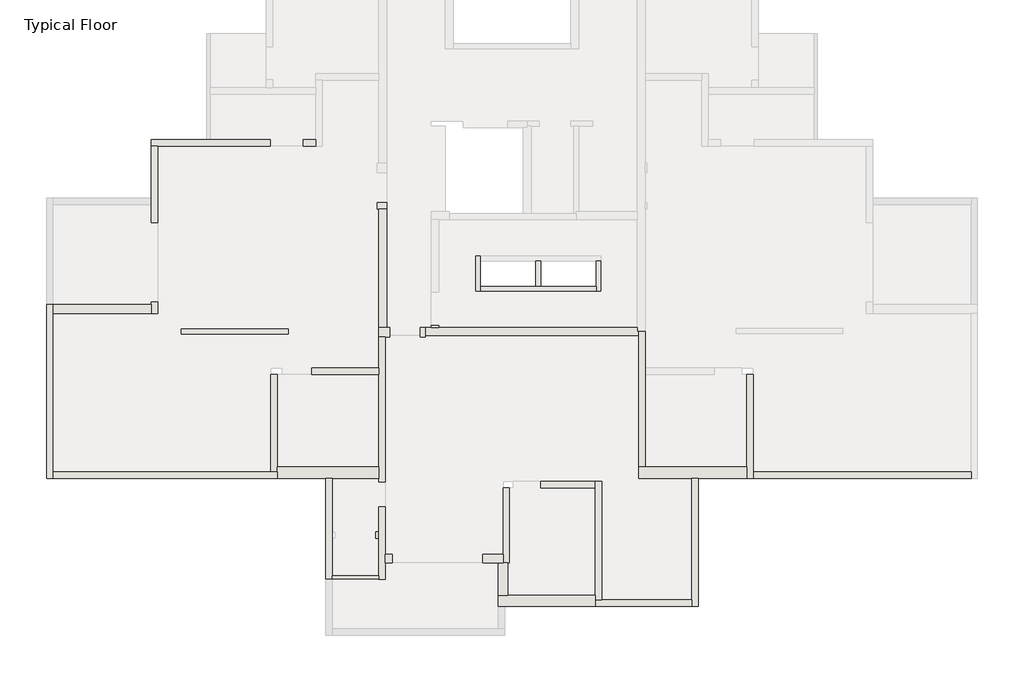
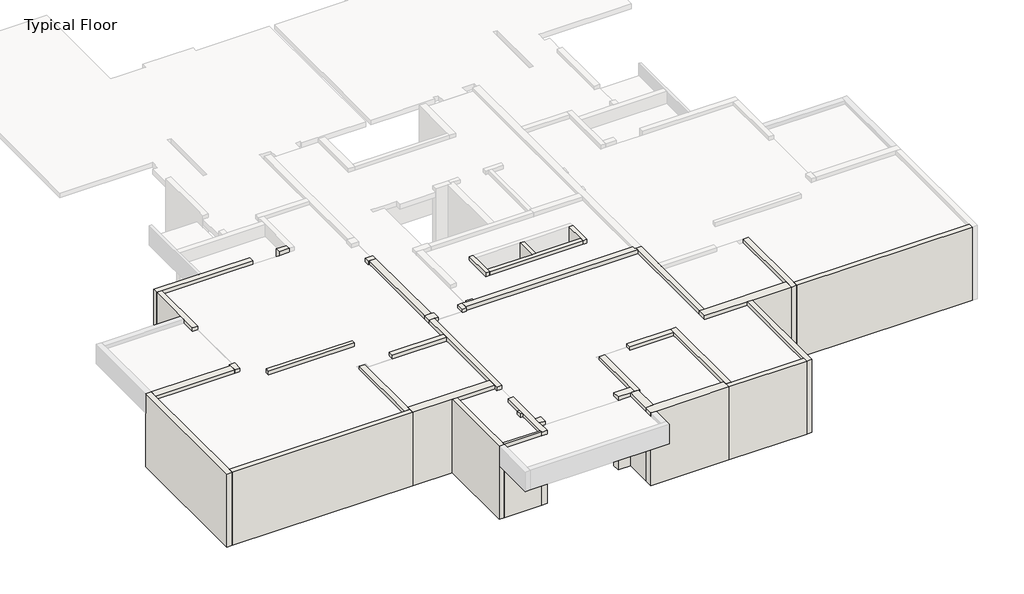
# One storey, part 1 of 4: 39 walls.
"""IFC4 building model written with IfcOpenShell, lengths in millimetres."""

from ifc_helpers import new_model, si_unit, frame, origin, place, context, project, spatial, polyline, outline, extrude, faceted_brep, element, save

model = new_model("IFC4")

# Units and contexts
model_context = context("Model", 3, world=origin())
ifc_project = project(units=[si_unit("LENGTHUNIT", "METRE", prefix="MILLI")], contexts=[model_context])

# Site, building, storey
site = spatial("IfcSite", under=ifc_project)
building = spatial("IfcBuilding", under=site)
storey = spatial("IfcBuildingStorey", under=building, Name="Typical Floor", Elevation=3160.0)

# Walls
placement = place(None, origin())
element("IfcWall", 1, ObjectType="10", at=placement, inside=storey, context=model_context, shape_type="Brep", body=[
    faceted_brep([(-1104.0660316, -14027.6329213, 160.0), (353.6524939, -14027.6329213, 160.0), (353.6524939, -14027.6329213, 2810.0), (353.6524939, -14027.6329213, 3010.0), (353.6524939, -14027.6329213, 3160.0), (-1104.0660316, -14027.6329213, 3160.0), (-1104.0660316, -14027.6329213, 3010.0), (-1104.0660316, -14027.6329213, 2810.0), (-1104.0660316, -13927.6329213, 160.0), (-1104.0660316, -13927.6329213, 3160.0), (353.6524939, -13927.6329213, 3160.0), (353.6524939, -13927.6329213, 3010.0), (353.6524939, -13927.6329213, 2810.0), (353.6524939, -13927.6329213, 160.0)], [[[0, 1, 2, 3, 4, 5, 6, 7]], [[8, 9, 10, 11, 12, 13]], [[1, 0, 8, 13]], [[5, 4, 10, 9]], [[4, 3, 2, 1, 13, 12, 11, 10]], [[0, 7, 6, 5, 9, 8]]]),
])
element("IfcWall", 2, ObjectType="15", at=placement, inside=storey, context=model_context, shape_type="Brep", body=[
    faceted_brep([(-5822.171691, -6349.5529829, 160.0), (-2483.2956212, -6349.5529829, 160.0), (-2483.2956212, -6349.5529829, 2810.0), (-2483.2956212, -6349.5529829, 3010.0), (-2483.2956212, -6349.5529829, 3160.0), (-5822.171691, -6349.5529829, 3160.0), (-5822.171691, -6349.5529829, 3010.0), (-5822.171691, -6349.5529829, 2810.0), (-5822.171691, -6199.5529829, 160.0), (-5822.171691, -6199.5529829, 2810.0), (-5822.171691, -6199.5529829, 3010.0), (-5822.171691, -6199.5529829, 3160.0), (-2483.2956212, -6199.5529829, 3160.0), (-2483.2956212, -6199.5529829, 3010.0), (-2483.2956212, -6199.5529829, 2810.0), (-2483.2956212, -6199.5529829, 160.0)], [[[0, 1, 2, 3, 4, 5, 6, 7]], [[8, 9, 10, 11, 12, 13, 14, 15]], [[1, 0, 8, 15]], [[4, 3, 2, 1, 15, 14, 13, 12]], [[5, 4, 12, 11]], [[0, 7, 6, 5, 11, 10, 9, 8]]]),
])
element("IfcWall", 3, ObjectType="15", at=placement, inside=storey, context=model_context, shape_type="Brep", body=[
    faceted_brep([(3535.5549057, -5009.2269053, 160.0), (3535.5549057, -4859.2269053, 160.0), (3535.5549057, -4065.4538564, 160.0), (3535.5549057, -3915.4538564, 160.0), (3535.5549057, -3915.4538564, 3160.0), (3535.5549057, -4065.4538564, 3160.0), (3535.5549057, -4859.2269053, 3160.0), (3535.5549057, -5009.2269053, 3160.0), (3385.5549057, -5009.2269053, 160.0), (3385.5549057, -5009.2269053, 2810.0), (3385.5549057, -5009.2269053, 3010.0), (3385.5549057, -5009.2269053, 3160.0), (3385.5549057, -3915.4538564, 3160.0), (3385.5549057, -3915.4538564, 3010.0), (3385.5549057, -3915.4538564, 2810.0), (3385.5549057, -3915.4538564, 160.0)], [[[0, 1, 2, 3, 4, 5, 6, 7]], [[8, 9, 10, 11, 12, 13, 14, 15]], [[3, 2, 1, 0, 8, 15]], [[7, 6, 5, 4, 12, 11]], [[4, 3, 15, 14, 13, 12]], [[0, 7, 11, 10, 9, 8]]]),
])
element("IfcWall", 4, ObjectType="15", at=placement, inside=storey, context=model_context, shape_type="Brep", body=[
    faceted_brep([(7154.2538596, -4065.4538564, 160.0), (7154.2538596, -4859.2269053, 160.0), (7154.2538596, -5009.2269053, 160.0), (7154.2538596, -5009.2269053, 3160.0), (7154.2538596, -4859.2269053, 3160.0), (7154.2538596, -4065.4538564, 3160.0), (7304.2538596, -4065.4538564, 160.0), (7304.2538596, -4065.4538564, 3160.0), (7304.2538596, -5009.2269053, 3160.0), (7304.2538596, -5009.2269053, 3010.0), (7304.2538596, -5009.2269053, 2810.0), (7304.2538596, -5009.2269053, 160.0)], [[[0, 1, 2, 3, 4, 5]], [[6, 7, 8, 9, 10, 11]], [[2, 1, 0, 6, 11]], [[5, 4, 3, 8, 7]], [[0, 5, 7, 6]], [[3, 2, 11, 10, 9, 8]]]),
])
element("IfcWall", 5, ObjectType="15", at=placement, inside=storey, context=model_context, shape_type="Brep", body=[
    faceted_brep([(7154.2538596, -4859.2269053, 160.0), (5418.6420666, -4859.2269053, 160.0), (5268.6420666, -4859.2269053, 160.0), (3535.5549057, -4859.2269053, 160.0), (3535.5549057, -4859.2269053, 3160.0), (5268.6420666, -4859.2269053, 3160.0), (5418.6420666, -4859.2269053, 3160.0), (7154.2538596, -4859.2269053, 3160.0), (7154.2538596, -5009.2269053, 160.0), (7154.2538596, -5009.2269053, 3160.0), (3535.5549057, -5009.2269053, 3160.0), (3535.5549057, -5009.2269053, 160.0)], [[[0, 1, 2, 3, 4, 5, 6, 7]], [[8, 9, 10, 11]], [[3, 2, 1, 0, 8, 11]], [[7, 6, 5, 4, 10, 9]], [[0, 7, 9, 8]], [[4, 3, 11, 10]]]),
])
element("IfcWall", 6, ObjectType="15", at=placement, inside=storey, context=model_context, shape_type="SweptSolid", body=[
    extrude(outline(polyline([(5418.6420666, -4065.4538564), (5418.6420666, -4859.2269053), (5268.6420666, -4859.2269053), (5268.6420666, -4065.4538564), (5418.6420666, -4065.4538564)])), frame((0.0, 0.0, 160.0), z_axis=(0.0, 0.0, 1.0), x_axis=(1.0, 0.0, 0.0)), (0.0, 0.0, 1.0), 3000.0),
])
element("IfcWall", 7, ObjectType="20", at=placement, inside=storey, context=model_context, shape_type="Brep", body=[
    faceted_brep([(10348.1730809, -14884.0133443, 160.0), (10348.1730809, -10869.1739201, 160.0), (10348.1730809, -10869.1739201, 3160.0), (10348.1730809, -14884.0133443, 3160.0), (10148.1730809, -14884.0133443, 160.0), (10148.1730809, -14884.0133443, 3160.0), (10148.1730809, -14684.0133443, 3160.0), (10148.1730809, -10869.1739201, 3160.0), (10148.1730809, -10869.1739201, 3010.0), (10148.1730809, -10869.1739201, 2810.0), (10148.1730809, -10869.1739201, 160.0), (10148.1730809, -14684.0133443, 160.0)], [[[0, 1, 2, 3]], [[4, 5, 6, 7, 8, 9, 10, 11]], [[1, 0, 4, 11, 10]], [[3, 2, 7, 6, 5]], [[2, 1, 10, 9, 8, 7]], [[0, 3, 5, 4]]]),
])
element("IfcWall", 8, ObjectType="20", at=placement, inside=storey, context=model_context, shape_type="Brep", body=[
    faceted_brep([(10148.1730809, -14684.0133443, 160.0), (7323.2436151, -14684.0133443, 160.0), (7123.2436151, -14684.0133443, 160.0), (7123.2436151, -14684.0133443, 3160.0), (7323.2436151, -14684.0133443, 3160.0), (10148.1730809, -14684.0133443, 3160.0), (10148.1730809, -14684.0133443, 3010.0), (10148.1730809, -14684.0133443, 2810.0), (10148.1730809, -14884.0133443, 160.0), (10148.1730809, -14884.0133443, 3160.0), (7123.2436151, -14884.0133443, 3160.0), (7123.2436151, -14884.0133443, 160.0)], [[[0, 1, 2, 3, 4, 5, 6, 7]], [[8, 9, 10, 11]], [[2, 1, 0, 8, 11]], [[5, 4, 3, 10, 9]], [[3, 2, 11, 10]], [[0, 7, 6, 5, 9, 8]]]),
])
element("IfcWall", 9, ObjectType="20", at=placement, inside=storey, context=model_context, shape_type="Brep", body=[
    faceted_brep([(7323.2436151, -14684.0133443, 160.0), (7323.2436151, -10973.6256761, 160.0), (7323.2436151, -10973.6256761, 2810.0), (7323.2436151, -10973.6256761, 3010.0), (7323.2436151, -10973.6256761, 3160.0), (7323.2436151, -14684.0133443, 3160.0), (7323.2436151, -14684.0133443, 3010.0), (7323.2436151, -14684.0133443, 2810.0), (7123.2436151, -14684.0133443, 160.0), (7123.2436151, -14684.0133443, 3160.0), (7123.2436151, -14534.0137597, 3160.0), (7123.2436151, -11173.6256761, 3160.0), (7123.2436151, -10973.6256761, 3160.0), (7123.2436151, -10973.6256761, 160.0), (7123.2436151, -11173.6256761, 160.0), (7123.2436151, -14534.0137597, 160.0)], [[[0, 1, 2, 3, 4, 5, 6, 7]], [[8, 9, 10, 11, 12, 13, 14, 15]], [[1, 0, 8, 15, 14, 13]], [[5, 4, 12, 11, 10, 9]], [[4, 3, 2, 1, 13, 12]], [[0, 7, 6, 5, 9, 8]]]),
])
element("IfcWall", 10, ObjectType="20", at=placement, inside=storey, context=model_context, shape_type="Brep", body=[
    faceted_brep([(7123.2436151, -10973.6256761, 160.0), (5423.2436151, -10973.6256761, 160.0), (5423.2436151, -10973.6256761, 2810.0), (5423.2436151, -10973.6256761, 3010.0), (5423.2436151, -10973.6256761, 3160.0), (7123.2436151, -10973.6256761, 3160.0), (7123.2436151, -11173.6256761, 160.0), (7123.2436151, -11173.6256761, 2810.0), (7123.2436151, -11173.6256761, 3010.0), (7123.2436151, -11173.6256761, 3160.0), (5423.2436151, -11173.6256761, 3160.0), (5423.2436151, -11173.6256761, 3010.0), (5423.2436151, -11173.6256761, 2810.0), (5423.2436151, -11173.6256761, 160.0)], [[[0, 1, 2, 3, 4, 5]], [[6, 7, 8, 9, 10, 11, 12, 13]], [[1, 0, 6, 13]], [[4, 3, 2, 1, 13, 12, 11, 10]], [[5, 4, 10, 9]], [[0, 5, 9, 8, 7, 6]]]),
])
element("IfcWall", 11, ObjectType="20", at=placement, inside=storey, context=model_context, shape_type="Brep", body=[
    faceted_brep([(4441.3412033, -13527.809147, 160.0), (4441.3412033, -11173.6256761, 160.0), (4441.3412033, -11173.6256761, 2810.0), (4441.3412033, -11173.6256761, 3010.0), (4441.3412033, -11173.6256761, 3160.0), (4441.3412033, -13527.809147, 3160.0), (4441.3412033, -13527.809147, 3010.0), (4441.3412033, -13527.809147, 2810.0), (4241.3412033, -13527.809147, 160.0), (4241.3412033, -13527.809147, 3160.0), (4241.3412033, -13247.809147, 3160.0), (4241.3412033, -11173.6256761, 3160.0), (4241.3412033, -11173.6256761, 160.0), (4241.3412033, -13247.809147, 160.0), (4393.8641143, -13527.809147, 160.0), (4393.8641143, -13527.809147, 3160.0)], [[[0, 1, 2, 3, 4, 5, 6, 7]], [[8, 9, 10, 11, 12, 13]], [[1, 0, 14, 8, 13, 12]], [[5, 4, 11, 10, 9, 15]], [[0, 7, 6, 5, 15, 9, 8, 14]], [[4, 3, 2, 1, 12, 11]]]),
])
element("IfcWall", 12, ObjectType="20", at=placement, inside=storey, context=model_context, shape_type="Brep", body=[
    faceted_brep([(18889.4302812, -10669.1739201, 160.0), (12069.8374389, -10669.1739201, 160.0), (12069.8374389, -10669.1739201, 2810.0), (12069.8374389, -10669.1739201, 3010.0), (12069.8374389, -10669.1739201, 3160.0), (18889.4302812, -10669.1739201, 3160.0), (18889.4302812, -10669.1739201, 3010.0), (18889.4302812, -10669.1739201, 2810.0), (18889.4302812, -10869.1739201, 160.0), (18889.4302812, -10869.1739201, 3160.0), (12069.8374389, -10869.1739201, 3160.0), (12069.8374389, -10869.1739201, 160.0)], [[[0, 1, 2, 3, 4, 5, 6, 7]], [[8, 9, 10, 11]], [[1, 0, 8, 11]], [[5, 4, 10, 9]], [[0, 7, 6, 5, 9, 8]], [[4, 3, 2, 1, 11, 10]]]),
])
element("IfcWall", 13, ObjectType="20", at=placement, inside=storey, context=model_context, shape_type="Brep", body=[
    faceted_brep([(11869.8374389, -7625.251138, 160.0), (11869.8374389, -10519.1739201, 160.0), (11869.8374389, -10869.1739201, 160.0), (11869.8374389, -10869.1739201, 3160.0), (11869.8374389, -10519.1739201, 3160.0), (11869.8374389, -7625.251138, 3160.0), (11869.8374389, -7625.251138, 3010.0), (11869.8374389, -7625.251138, 2810.0), (12069.8374389, -7625.251138, 160.0), (12069.8374389, -7625.251138, 3160.0), (12069.8374389, -10669.1739201, 3160.0), (12069.8374389, -10869.1739201, 3160.0), (12069.8374389, -10869.1739201, 160.0), (12069.8374389, -10669.1739201, 160.0)], [[[0, 1, 2, 3, 4, 5, 6, 7]], [[8, 9, 10, 11, 12, 13]], [[2, 1, 0, 8, 13, 12]], [[5, 4, 3, 11, 10, 9]], [[3, 2, 12, 11]], [[0, 7, 6, 5, 9, 8]]]),
])
element("IfcWall", 14, ObjectType="20", at=placement, inside=storey, context=model_context, shape_type="Brep", body=[
    faceted_brep([(8689.2361919, -10519.1739201, 160.0), (8689.2361919, -7625.251138, 160.0), (8689.2361919, -7425.251138, 160.0), (8689.2361919, -6275.4733638, 160.0), (8689.2361919, -6275.4733638, 3160.0), (8689.2361919, -7425.251138, 3160.0), (8689.2361919, -7625.251138, 3160.0), (8689.2361919, -10519.1739201, 3160.0), (8689.2361919, -10519.1739201, 3010.0), (8689.2361919, -10519.1739201, 2810.0), (8489.2361919, -10519.1739201, 160.0), (8489.2361919, -10519.1739201, 3160.0), (8489.2361919, -6400.4733638, 3160.0), (8489.2361919, -6275.4733638, 3160.0), (8489.2361919, -6275.4733638, 160.0), (8489.2361919, -6400.4733638, 160.0)], [[[0, 1, 2, 3, 4, 5, 6, 7, 8, 9]], [[10, 11, 12, 13, 14, 15]], [[3, 2, 1, 0, 10, 15, 14]], [[4, 3, 14, 13]], [[7, 6, 5, 4, 13, 12, 11]], [[0, 9, 8, 7, 11, 10]]]),
])
element("IfcWall", 15, ObjectType="20", at=placement, inside=storey, context=model_context, shape_type="Brep", body=[
    faceted_brep([(-3044.013165, -271.5347538, 160.0), (-6764.013165, -271.5347538, 160.0), (-6764.013165, -271.5347538, 3160.0), (-3044.013165, -271.5347538, 3160.0), (-3044.013165, -271.5347538, 2660.0), (-3044.013165, -271.5347538, 2510.0), (-3044.013165, -471.5347538, 160.0), (-3044.013165, -471.5347538, 2510.0), (-3044.013165, -471.5347538, 2660.0), (-3044.013165, -471.5347538, 3160.0), (-6564.013165, -471.5347538, 3160.0), (-6764.013165, -471.5347538, 3160.0), (-6764.013165, -471.5347538, 160.0), (-6564.013165, -471.5347538, 160.0)], [[[0, 1, 2, 3, 4, 5]], [[6, 7, 8, 9, 10, 11, 12, 13]], [[1, 0, 6, 13, 12]], [[3, 2, 11, 10, 9]], [[0, 5, 4, 3, 9, 8, 7, 6]], [[2, 1, 12, 11]]]),
])
element("IfcWall", 16, ObjectType="20", at=placement, inside=storey, context=model_context, shape_type="Brep", body=[
    faceted_brep([(-10045.3223417, -5427.6243159, 160.0), (-10045.3223417, -10869.1739201, 160.0), (-10045.3223417, -10869.1739201, 3160.0), (-10045.3223417, -5427.6243159, 3160.0), (-9845.3223417, -5427.6243159, 160.0), (-9845.3223417, -5427.6243159, 3160.0), (-9845.3223417, -5707.6243159, 3160.0), (-9845.3223417, -10669.1739201, 3160.0), (-9845.3223417, -10869.1739201, 3160.0), (-9845.3223417, -10869.1739201, 160.0), (-9845.3223417, -10669.1739201, 160.0), (-9845.3223417, -5707.6243159, 160.0)], [[[0, 1, 2, 3]], [[4, 5, 6, 7, 8, 9, 10, 11]], [[1, 0, 4, 11, 10, 9]], [[3, 2, 8, 7, 6, 5]], [[2, 1, 9, 8]], [[0, 3, 5, 4]]]),
])
element("IfcWall", 17, ObjectType="20", at=placement, inside=storey, context=model_context, shape_type="Brep", body=[
    faceted_brep([(-9845.3223417, -10869.1739201, 160.0), (-2825.3223417, -10869.1739201, 160.0), (-2825.3223417, -10869.1739201, 3160.0), (-9845.3223417, -10869.1739201, 3160.0), (-9845.3223417, -10669.1739201, 160.0), (-9845.3223417, -10669.1739201, 2810.0), (-9845.3223417, -10669.1739201, 3010.0), (-9845.3223417, -10669.1739201, 3160.0), (-3025.7294994, -10669.1739201, 3160.0), (-2825.7294994, -10669.1739201, 3160.0), (-2825.3223417, -10669.1739201, 3160.0), (-2825.3223417, -10669.1739201, 160.0), (-2825.7294994, -10669.1739201, 160.0), (-3025.7294994, -10669.1739201, 160.0)], [[[0, 1, 2, 3]], [[4, 5, 6, 7, 8, 9, 10, 11, 12, 13]], [[1, 0, 4, 13, 12, 11]], [[2, 1, 11, 10]], [[3, 2, 10, 9, 8, 7]], [[0, 3, 7, 6, 5, 4]]]),
])
element("IfcWall", 18, ObjectType="20", at=placement, inside=storey, context=model_context, shape_type="Brep", body=[
    faceted_brep([(-3025.7294994, -7625.251138, 3160.0), (-3025.7294994, -7625.251138, 160.0), (-3025.7294994, -10669.1739201, 160.0), (-3025.7294994, -10669.1739201, 2810.0), (-3025.7294994, -10669.1739201, 3010.0), (-3025.7294994, -10669.1739201, 3160.0), (-2825.7294994, -7625.251138, 160.0), (-2825.7294994, -7625.251138, 2810.0), (-2825.7294994, -7625.251138, 3010.0), (-2825.7294994, -7625.251138, 3160.0), (-2825.7294994, -10519.1739201, 3160.0), (-2825.7294994, -10669.1739201, 3160.0), (-2825.7294994, -10669.1739201, 160.0), (-2825.7294994, -10519.1739201, 160.0)], [[[0, 1, 2, 3, 4, 5]], [[6, 7, 8, 9, 10, 11, 12, 13]], [[1, 6, 13, 12, 2]], [[9, 0, 5, 11, 10]], [[5, 4, 3, 2, 12, 11]], [[1, 0, 9, 8, 7, 6]]]),
])
element("IfcWall", 19, ObjectType="20", at=placement, inside=storey, context=model_context, shape_type="Brep", body=[
    faceted_brep([(-1746.3475061, -7625.251138, 160.0), (353.6524939, -7625.251138, 160.0), (353.6524939, -7625.251138, 2810.0), (353.6524939, -7625.251138, 3010.0), (353.6524939, -7625.251138, 3160.0), (-1746.3475061, -7625.251138, 3160.0), (-1746.3475061, -7625.251138, 3010.0), (-1746.3475061, -7625.251138, 2810.0), (-1746.3475061, -7425.251138, 160.0), (-1746.3475061, -7425.251138, 2810.0), (-1746.3475061, -7425.251138, 3010.0), (-1746.3475061, -7425.251138, 3160.0), (353.6524939, -7425.251138, 3160.0), (353.6524939, -7425.251138, 3010.0), (353.6524939, -7425.251138, 2810.0), (353.6524939, -7425.251138, 160.0)], [[[0, 1, 2, 3, 4, 5, 6, 7]], [[8, 9, 10, 11, 12, 13, 14, 15]], [[1, 0, 8, 15]], [[5, 4, 12, 11]], [[0, 7, 6, 5, 11, 10, 9, 8]], [[4, 3, 2, 1, 15, 14, 13, 12]]]),
])
element("IfcWall", 20, ObjectType="20", at=placement, inside=storey, context=model_context, shape_type="Brep", body=[
    faceted_brep([(353.6524939, -6450.4733638, 160.0), (353.6524939, -7425.251138, 160.0), (353.6524939, -7625.251138, 160.0), (353.6524939, -10519.1739201, 160.0), (353.6524939, -10869.1739201, 160.0), (353.6524939, -10989.1739201, 160.0), (353.6524939, -10989.1739201, 2810.0), (353.6524939, -10989.1739201, 3010.0), (353.6524939, -10989.1739201, 3160.0), (353.6524939, -10869.1739201, 3160.0), (353.6524939, -10519.1739201, 3160.0), (353.6524939, -7625.251138, 3160.0), (353.6524939, -7425.251138, 3160.0), (353.6524939, -6450.4733638, 3160.0), (553.6524939, -6450.4733638, 160.0), (553.6524939, -6450.4733638, 2810.0), (553.6524939, -6450.4733638, 3010.0), (553.6524939, -6450.4733638, 3160.0), (553.6524939, -10989.1739201, 3160.0), (553.6524939, -10989.1739201, 3010.0), (553.6524939, -10989.1739201, 2810.0), (553.6524939, -10989.1739201, 160.0)], [[[0, 1, 2, 3, 4, 5, 6, 7, 8, 9, 10, 11, 12, 13]], [[14, 15, 16, 17, 18, 19, 20, 21]], [[5, 4, 3, 2, 1, 0, 14, 21]], [[8, 7, 6, 5, 21, 20, 19, 18]], [[13, 12, 11, 10, 9, 8, 18, 17]], [[0, 13, 17, 16, 15, 14]]]),
])
element("IfcWall", 21, ObjectType="20", at=placement, inside=storey, context=model_context, shape_type="Brep", body=[
    faceted_brep([(553.6524939, -14034.1739201, 160.0), (553.6524939, -13527.809147, 160.0), (553.6524939, -13247.809147, 160.0), (553.6524939, -11774.1739201, 160.0), (553.6524939, -11774.1739201, 2810.0), (553.6524939, -11774.1739201, 3010.0), (553.6524939, -11774.1739201, 3160.0), (553.6524939, -13247.809147, 3160.0), (553.6524939, -13527.809147, 3160.0), (553.6524939, -14034.1739201, 3160.0), (553.6524939, -14034.1739201, 3010.0), (553.6524939, -14034.1739201, 2810.0), (353.6524939, -14034.1739201, 160.0), (353.6524939, -14034.1739201, 2810.0), (353.6524939, -14034.1739201, 3010.0), (353.6524939, -14034.1739201, 3160.0), (353.6524939, -14027.6329213, 3160.0), (353.6524939, -13927.6329213, 3160.0), (353.6524939, -12752.8550877, 3160.0), (353.6524939, -12552.8550877, 3160.0), (353.6524939, -11774.1739201, 3160.0), (353.6524939, -11774.1739201, 3010.0), (353.6524939, -11774.1739201, 2810.0), (353.6524939, -11774.1739201, 160.0), (353.6524939, -12552.8550877, 160.0), (353.6524939, -12752.8550877, 160.0), (353.6524939, -13927.6329213, 160.0), (353.6524939, -14027.6329213, 160.0)], [[[0, 1, 2, 3, 4, 5, 6, 7, 8, 9, 10, 11]], [[12, 13, 14, 15, 16, 17, 18, 19, 20, 21, 22, 23, 24, 25, 26, 27]], [[3, 2, 1, 0, 12, 27, 26, 25, 24, 23]], [[6, 5, 4, 3, 23, 22, 21, 20]], [[9, 8, 7, 6, 20, 19, 18, 17, 16, 15]], [[0, 11, 10, 9, 15, 14, 13, 12]]]),
])
element("IfcWall", 22, ObjectType="20", at=placement, inside=storey, context=model_context, shape_type="Brep", body=[
    faceted_brep([(-1304.0660316, -10869.1739201, 160.0), (-1304.0660316, -14027.6329213, 160.0), (-1304.0660316, -14027.6329213, 3160.0), (-1304.0660316, -10869.1739201, 3160.0), (-1104.0660316, -10869.1739201, 160.0), (-1104.0660316, -10869.1739201, 2810.0), (-1104.0660316, -10869.1739201, 3010.0), (-1104.0660316, -10869.1739201, 3160.0), (-1104.0660316, -12552.855147, 3160.0), (-1104.0660316, -12752.855147, 3160.0), (-1104.0660316, -13927.6329213, 3160.0), (-1104.0660316, -14027.6329213, 3160.0), (-1104.0660316, -14027.6329213, 160.0), (-1104.0660316, -13927.6329213, 160.0)], [[[0, 1, 2, 3]], [[4, 5, 6, 7, 8, 9, 10, 11, 12, 13]], [[1, 0, 4, 13, 12]], [[3, 2, 11, 10, 9, 8, 7]], [[0, 3, 7, 6, 5, 4]], [[2, 1, 12, 11]]]),
])
element("IfcWall", 23, ObjectType="20", at=placement, inside=storey, context=model_context, shape_type="Brep", body=[
    faceted_brep([(253.6524939, -12752.8550877, 160.0), (353.6524939, -12752.8550877, 160.0), (353.6524939, -12752.8550877, 2810.0), (353.6524939, -12752.8550877, 3010.0), (353.6524939, -12752.8550877, 3160.0), (253.6524939, -12752.8550877, 3160.0), (253.6524939, -12752.8550877, 3010.0), (253.6524939, -12752.8550877, 2810.0), (253.6524939, -12552.8550877, 160.0), (253.6524939, -12552.8550877, 2810.0), (253.6524939, -12552.8550877, 3010.0), (253.6524939, -12552.8550877, 3160.0), (353.6524939, -12552.8550877, 3160.0), (353.6524939, -12552.8550877, 3010.0), (353.6524939, -12552.8550877, 2810.0), (353.6524939, -12552.8550877, 160.0)], [[[0, 1, 2, 3, 4, 5, 6, 7]], [[8, 9, 10, 11, 12, 13, 14, 15]], [[1, 0, 8, 15]], [[5, 4, 12, 11]], [[0, 7, 6, 5, 11, 10, 9, 8]], [[4, 3, 2, 1, 15, 14, 13, 12]]]),
])
element("IfcWall", 24, ObjectType="20", at=placement, inside=storey, context=model_context, shape_type="Brep", body=[
    faceted_brep([(-6564.013165, -5707.6243159, 160.0), (-6564.013165, -5351.6580536, 160.0), (-6564.013165, -5351.6580536, 2810.0), (-6564.013165, -5351.6580536, 3010.0), (-6564.013165, -5351.6580536, 3160.0), (-6564.013165, -5707.6243159, 3160.0), (-6564.013165, -5707.6243159, 3010.0), (-6564.013165, -5707.6243159, 2810.0), (-6764.013165, -5707.6243159, 160.0), (-6764.013165, -5707.6243159, 3160.0), (-6764.013165, -5427.6243159, 3160.0), (-6764.013165, -5351.6580536, 3160.0), (-6764.013165, -5351.6580536, 3010.0), (-6764.013165, -5351.6580536, 2810.0), (-6764.013165, -5351.6580536, 160.0), (-6764.013165, -5427.6243159, 160.0)], [[[0, 1, 2, 3, 4, 5, 6, 7]], [[8, 9, 10, 11, 12, 13, 14, 15]], [[1, 0, 8, 15, 14]], [[4, 3, 2, 1, 14, 13, 12, 11]], [[5, 4, 11, 10, 9]], [[0, 7, 6, 5, 9, 8]]]),
])
element("IfcWall", 25, ObjectType="20", at=placement, inside=storey, context=model_context, shape_type="Brep", body=[
    faceted_brep([(-6564.013165, -2868.5711301, 160.0), (-6564.013165, -471.5347538, 160.0), (-6564.013165, -471.5347538, 2810.0), (-6564.013165, -471.5347538, 3010.0), (-6564.013165, -471.5347538, 3160.0), (-6564.013165, -2868.5711301, 3160.0), (-6564.013165, -2868.5711301, 3010.0), (-6564.013165, -2868.5711301, 2810.0), (-6764.013165, -2868.5711301, 160.0), (-6764.013165, -2868.5711301, 2810.0), (-6764.013165, -2868.5711301, 3010.0), (-6764.013165, -2868.5711301, 3160.0), (-6764.013165, -471.5347538, 3160.0), (-6764.013165, -471.5347538, 160.0)], [[[0, 1, 2, 3, 4, 5, 6, 7]], [[8, 9, 10, 11, 12, 13]], [[1, 0, 8, 13]], [[5, 4, 12, 11]], [[0, 7, 6, 5, 11, 10, 9, 8]], [[4, 3, 2, 1, 13, 12]]]),
])
element("IfcWall", 26, ObjectType="20", at=placement, inside=storey, context=model_context, shape_type="Brep", body=[
    faceted_brep([(303.6507728, -2440.6761415, 160.0), (353.6524939, -2440.6761415, 160.0), (603.6524939, -2440.6761415, 160.0), (603.6524939, -2440.6761415, 3160.0), (353.6524939, -2440.6761415, 3160.0), (303.6507728, -2440.6761415, 3160.0), (303.6507728, -2440.6761415, 3010.0), (303.6507728, -2440.6761415, 2810.0), (303.6507728, -2240.6761415, 160.0), (303.6507728, -2240.6761415, 2810.0), (303.6507728, -2240.6761415, 3010.0), (303.6507728, -2240.6761415, 3160.0), (603.6524939, -2240.6761415, 3160.0), (603.6524939, -2240.6761415, 3010.0), (603.6524939, -2240.6761415, 2810.0), (603.6524939, -2240.6761415, 160.0)], [[[0, 1, 2, 3, 4, 5, 6, 7]], [[8, 9, 10, 11, 12, 13, 14, 15]], [[2, 1, 0, 8, 15]], [[5, 4, 3, 12, 11]], [[0, 7, 6, 5, 11, 10, 9, 8]], [[3, 2, 15, 14, 13, 12]]]),
])
element("IfcWall", 27, ObjectType="20", at=placement, inside=storey, context=model_context, shape_type="Brep", body=[
    faceted_brep([(-1618.0126357, -271.5347538, 160.0), (-2018.0126357, -271.5347538, 160.0), (-2018.0126357, -271.5347538, 2510.0), (-2018.0126357, -271.5347538, 2660.0), (-2018.0126357, -271.5347538, 3160.0), (-1618.0126357, -271.5347538, 3160.0), (-1618.0126357, -271.5347538, 2660.0), (-1618.0126357, -271.5347538, 2510.0), (-1618.0126357, -471.5347538, 160.0), (-1618.0126357, -471.5347538, 3160.0), (-2018.0126357, -471.5347538, 3160.0), (-2018.0126357, -471.5347538, 2660.0), (-2018.0126357, -471.5347538, 2510.0), (-2018.0126357, -471.5347538, 160.0)], [[[0, 1, 2, 3, 4, 5, 6, 7]], [[8, 9, 10, 11, 12, 13]], [[1, 0, 8, 13]], [[4, 3, 2, 1, 13, 12, 11, 10]], [[5, 4, 10, 9]], [[0, 7, 6, 5, 9, 8]]]),
])
element("IfcWall", 28, ObjectType="25", at=placement, inside=storey, context=model_context, shape_type="Brep", body=[
    faceted_brep([(353.6524939, -2440.6761415, 160.0), (353.6524939, -6150.4733638, 160.0), (353.6524939, -6150.4733638, 3160.0), (353.6524939, -2440.6761415, 3160.0), (353.6524939, -2440.6761415, 3010.0), (353.6524939, -2440.6761415, 2810.0), (603.6524939, -2440.6761415, 160.0), (603.6524939, -2440.6761415, 3160.0), (603.6524939, -6150.4733638, 3160.0), (603.6524939, -6150.4733638, 3010.0), (603.6524939, -6150.4733638, 2810.0), (603.6524939, -6150.4733638, 160.0)], [[[0, 1, 2, 3, 4, 5]], [[6, 7, 8, 9, 10, 11]], [[1, 0, 6, 11]], [[3, 2, 8, 7]], [[2, 1, 11, 10, 9, 8]], [[0, 5, 4, 3, 7, 6]]]),
])
element("IfcWall", 29, ObjectType="25", at=placement, inside=storey, context=model_context, shape_type="Brep", body=[
    faceted_brep([(1804.8990117, -6400.4733638, 160.0), (8489.2361919, -6400.4733638, 160.0), (8489.2361919, -6400.4733638, 2810.0), (8489.2361919, -6400.4733638, 3010.0), (8489.2361919, -6400.4733638, 3160.0), (1804.8990117, -6400.4733638, 3160.0), (1804.8990117, -6400.4733638, 3010.0), (1804.8990117, -6400.4733638, 2810.0), (1804.8990117, -6150.4733638, 160.0), (1804.8990117, -6150.4733638, 3160.0), (1987.3338395, -6150.4733638, 3160.0), (2237.3338395, -6150.4733638, 3160.0), (8439.2361919, -6150.4733638, 3160.0), (8439.2361919, -6150.4733638, 3010.0), (8439.2361919, -6150.4733638, 2810.0), (8439.2361919, -6150.4733638, 160.0), (2237.3338395, -6150.4733638, 160.0), (1987.3338395, -6150.4733638, 160.0), (8439.2361919, -6275.4733638, 160.0), (8489.2361919, -6275.4733638, 160.0), (8489.2361919, -6275.4733638, 3160.0), (8439.2361919, -6275.4733638, 3160.0)], [[[0, 1, 2, 3, 4, 5, 6, 7]], [[8, 9, 10, 11, 12, 13, 14, 15, 16, 17]], [[1, 0, 8, 17, 16, 15, 18, 19]], [[5, 4, 20, 21, 12, 11, 10, 9]], [[0, 7, 6, 5, 9, 8]], [[4, 3, 2, 1, 19, 20]], [[19, 18, 21, 20]], [[18, 15, 14, 13, 12, 21]]]),
])
element("IfcWall", 30, ObjectType="25", at=placement, inside=storey, context=model_context, shape_type="Brep", body=[
    faceted_brep([(1987.3338395, -6084.0047389, 160.0), (1987.3338395, -6150.4733638, 160.0), (1987.3338395, -6150.4733638, 2810.0), (1987.3338395, -6150.4733638, 3010.0), (1987.3338395, -6150.4733638, 3160.0), (1987.3338395, -6084.0047389, 3160.0), (1987.3338395, -6084.0047389, 3010.0), (1987.3338395, -6084.0047389, 2810.0), (2237.3338395, -6084.0047389, 160.0), (2237.3338395, -6084.0047389, 2810.0), (2237.3338395, -6084.0047389, 3010.0), (2237.3338395, -6084.0047389, 3160.0), (2237.3338395, -6150.4733638, 3160.0), (2237.3338395, -6150.4733638, 3010.0), (2237.3338395, -6150.4733638, 2810.0), (2237.3338395, -6150.4733638, 160.0)], [[[0, 1, 2, 3, 4, 5, 6, 7]], [[8, 9, 10, 11, 12, 13, 14, 15]], [[1, 0, 8, 15]], [[5, 4, 12, 11]], [[0, 7, 6, 5, 11, 10, 9, 8]], [[4, 3, 2, 1, 15, 14, 13, 12]]]),
])
element("IfcWall", 31, ObjectType="28", at=placement, inside=storey, context=model_context, shape_type="Brep", body=[
    faceted_brep([(4241.3412033, -13247.809147, 160.0), (3603.9523756, -13247.809147, 160.0), (3603.9523756, -13247.809147, 2810.0), (3603.9523756, -13247.809147, 3010.0), (3603.9523756, -13247.809147, 3160.0), (4241.3412033, -13247.809147, 3160.0), (4241.3412033, -13247.809147, 3010.0), (4241.3412033, -13247.809147, 2810.0), (4241.3412033, -13527.809147, 160.0), (4241.3412033, -13527.809147, 3160.0), (4093.8641143, -13527.809147, 3160.0), (3603.9523756, -13527.809147, 3160.0), (3603.9523756, -13527.809147, 3010.0), (3603.9523756, -13527.809147, 2810.0), (3603.9523756, -13527.809147, 160.0), (4093.8641143, -13527.809147, 160.0)], [[[0, 1, 2, 3, 4, 5, 6, 7]], [[8, 9, 10, 11, 12, 13, 14, 15]], [[1, 0, 8, 15, 14]], [[4, 3, 2, 1, 14, 13, 12, 11]], [[5, 4, 11, 10, 9]], [[0, 7, 6, 5, 9, 8]]]),
])
element("IfcWall", 32, ObjectType="28", at=placement, inside=storey, context=model_context, shape_type="Brep", body=[
    faceted_brep([(-6764.013165, -5427.6243159, 160.0), (-9845.3223417, -5427.6243159, 160.0), (-9845.3223417, -5427.6243159, 2810.0), (-9845.3223417, -5427.6243159, 3010.0), (-9845.3223417, -5427.6243159, 3160.0), (-6764.013165, -5427.6243159, 3160.0), (-6764.013165, -5427.6243159, 3010.0), (-6764.013165, -5427.6243159, 2810.0), (-6764.013165, -5707.6243159, 160.0), (-6764.013165, -5707.6243159, 3160.0), (-9845.3223417, -5707.6243159, 3160.0), (-9845.3223417, -5707.6243159, 3010.0), (-9845.3223417, -5707.6243159, 2810.0), (-9845.3223417, -5707.6243159, 160.0)], [[[0, 1, 2, 3, 4, 5, 6, 7]], [[8, 9, 10, 11, 12, 13]], [[1, 0, 8, 13]], [[5, 4, 10, 9]], [[0, 7, 6, 5, 9, 8]], [[4, 3, 2, 1, 13, 12, 11, 10]]]),
])
element("IfcWall", 33, ObjectType="28", at=placement, inside=storey, context=model_context, shape_type="Brep", body=[
    faceted_brep([(553.6524939, -13527.809147, 160.0), (769.5270528, -13527.809147, 160.0), (769.5270528, -13527.809147, 2810.0), (769.5270528, -13527.809147, 3010.0), (769.5270528, -13527.809147, 3160.0), (553.6524939, -13527.809147, 3160.0), (553.6524939, -13527.809147, 3010.0), (553.6524939, -13527.809147, 2810.0), (553.6524939, -13247.809147, 160.0), (553.6524939, -13247.809147, 2810.0), (553.6524939, -13247.809147, 3010.0), (553.6524939, -13247.809147, 3160.0), (769.5270528, -13247.809147, 3160.0), (769.5270528, -13247.809147, 3010.0), (769.5270528, -13247.809147, 2810.0), (769.5270528, -13247.809147, 160.0)], [[[0, 1, 2, 3, 4, 5, 6, 7]], [[8, 9, 10, 11, 12, 13, 14, 15]], [[1, 0, 8, 15]], [[4, 3, 2, 1, 15, 14, 13, 12]], [[5, 4, 12, 11]], [[0, 7, 6, 5, 11, 10, 9, 8]]]),
])
element("IfcWall", 34, ObjectType="30", at=placement, inside=storey, context=model_context, shape_type="Brep", body=[
    faceted_brep([(4093.8641143, -13527.809147, 160.0), (4093.8641143, -14534.0137597, 160.0), (4093.8641143, -14534.0137597, 3160.0), (4093.8641143, -13527.809147, 3160.0), (4093.8641143, -13527.809147, 3010.0), (4093.8641143, -13527.809147, 2810.0), (4393.8641143, -13527.809147, 160.0), (4393.8641143, -13527.809147, 2810.0), (4393.8641143, -13527.809147, 3010.0), (4393.8641143, -13527.809147, 3160.0), (4393.8641143, -14534.0137597, 3160.0), (4393.8641143, -14534.0137597, 160.0), (4241.3412033, -13527.809147, 160.0), (4241.3412033, -13527.809147, 3160.0)], [[[0, 1, 2, 3, 4, 5]], [[6, 7, 8, 9, 10, 11]], [[1, 0, 12, 6, 11]], [[3, 2, 10, 9, 13]], [[2, 1, 11, 10]], [[0, 5, 4, 3, 13, 9, 8, 7, 6, 12]]]),
])
element("IfcWall", 35, ObjectType="30", at=placement, inside=storey, context=model_context, shape_type="Brep", body=[
    faceted_brep([(353.6524939, -6450.4733638, 160.0), (553.6524939, -6450.4733638, 160.0), (703.0584279, -6450.4733638, 160.0), (703.0584279, -6450.4733638, 2810.0), (703.0584279, -6450.4733638, 3010.0), (703.0584279, -6450.4733638, 3160.0), (553.6524939, -6450.4733638, 3160.0), (353.6524939, -6450.4733638, 3160.0), (353.6524939, -6150.4733638, 160.0), (353.6524939, -6150.4733638, 3160.0), (603.6524939, -6150.4733638, 3160.0), (703.0584279, -6150.4733638, 3160.0), (703.0584279, -6150.4733638, 3010.0), (703.0584279, -6150.4733638, 2810.0), (703.0584279, -6150.4733638, 160.0), (603.6524939, -6150.4733638, 160.0)], [[[0, 1, 2, 3, 4, 5, 6, 7]], [[8, 9, 10, 11, 12, 13, 14, 15]], [[2, 1, 0, 8, 15, 14]], [[5, 4, 3, 2, 14, 13, 12, 11]], [[7, 6, 5, 11, 10, 9]], [[0, 7, 9, 8]]]),
])
element("IfcWall", 36, ObjectType="30", at=placement, inside=storey, context=model_context, shape_type="Brep", body=[
    faceted_brep([(1644.8990117, -6450.4733638, 160.0), (1804.8990117, -6450.4733638, 160.0), (1804.8990117, -6450.4733638, 2810.0), (1804.8990117, -6450.4733638, 3010.0), (1804.8990117, -6450.4733638, 3160.0), (1644.8990117, -6450.4733638, 3160.0), (1644.8990117, -6450.4733638, 3010.0), (1644.8990117, -6450.4733638, 2810.0), (1644.8990117, -6150.4733638, 160.0), (1644.8990117, -6150.4733638, 2810.0), (1644.8990117, -6150.4733638, 3010.0), (1644.8990117, -6150.4733638, 3160.0), (1804.8990117, -6150.4733638, 3160.0), (1804.8990117, -6150.4733638, 160.0), (1804.8990117, -6400.4733638, 160.0), (1804.8990117, -6400.4733638, 3160.0)], [[[0, 1, 2, 3, 4, 5, 6, 7]], [[8, 9, 10, 11, 12, 13]], [[1, 0, 8, 13, 14]], [[4, 3, 2, 1, 14, 13, 12, 15]], [[5, 4, 15, 12, 11]], [[0, 7, 6, 5, 11, 10, 9, 8]]]),
])
element("IfcWall", 37, ObjectType="35", at=placement, inside=storey, context=model_context, shape_type="Brep", body=[
    faceted_brep([(4093.8641143, -14884.0137597, 160.0), (7123.2436151, -14884.0137597, 160.0), (7123.2436151, -14884.0137597, 3160.0), (4293.8641143, -14884.0137597, 3160.0), (4093.8641143, -14884.0137597, 3160.0), (4093.8641143, -14884.0137597, 2360.0), (4093.8641143, -14534.0137597, 160.0), (4093.8641143, -14534.0137597, 3160.0), (4393.8641143, -14534.0137597, 3160.0), (7123.2436151, -14534.0137597, 3160.0), (7123.2436151, -14534.0137597, 3010.0), (7123.2436151, -14534.0137597, 2810.0), (7123.2436151, -14534.0137597, 160.0), (4393.8641143, -14534.0137597, 160.0), (7123.2436151, -14684.0133443, 160.0), (7123.2436151, -14684.0133443, 3160.0)], [[[0, 1, 2, 3, 4, 5]], [[6, 7, 8, 9, 10, 11, 12, 13]], [[1, 0, 6, 13, 12, 14]], [[4, 3, 2, 15, 9, 8, 7]], [[0, 5, 4, 7, 6]], [[2, 1, 14, 12, 11, 10, 9, 15]]]),
])
element("IfcWall", 38, ObjectType="35", at=placement, inside=storey, context=model_context, shape_type="Brep", body=[
    faceted_brep([(11869.8374389, -10519.1739201, 160.0), (8689.2361919, -10519.1739201, 160.0), (8489.2361919, -10519.1739201, 160.0), (8489.2361919, -10519.1739201, 3160.0), (8689.2361919, -10519.1739201, 3160.0), (11869.8374389, -10519.1739201, 3160.0), (11869.8374389, -10519.1739201, 3010.0), (11869.8374389, -10519.1739201, 2810.0), (11869.8374389, -10869.1739201, 160.0), (11869.8374389, -10869.1739201, 3160.0), (10348.1730809, -10869.1739201, 3160.0), (10148.1730809, -10869.1739201, 3160.0), (8489.2361919, -10869.1739201, 3160.0), (8489.2361919, -10869.1739201, 3010.0), (8489.2361919, -10869.1739201, 2810.0), (8489.2361919, -10869.1739201, 160.0), (10148.1730809, -10869.1739201, 160.0), (10348.1730809, -10869.1739201, 160.0)], [[[0, 1, 2, 3, 4, 5, 6, 7]], [[8, 9, 10, 11, 12, 13, 14, 15, 16, 17]], [[2, 1, 0, 8, 17, 16, 15]], [[5, 4, 3, 12, 11, 10, 9]], [[0, 7, 6, 5, 9, 8]], [[3, 2, 15, 14, 13, 12]]]),
])
element("IfcWall", 39, ObjectType="35", at=placement, inside=storey, context=model_context, shape_type="Brep", body=[
    faceted_brep([(353.6524939, -10519.1739201, 160.0), (-2825.7294994, -10519.1739201, 160.0), (-2825.7294994, -10519.1739201, 2810.0), (-2825.7294994, -10519.1739201, 3010.0), (-2825.7294994, -10519.1739201, 3160.0), (353.6524939, -10519.1739201, 3160.0), (353.6524939, -10519.1739201, 3010.0), (353.6524939, -10519.1739201, 2810.0), (353.6524939, -10869.1739201, 160.0), (353.6524939, -10869.1739201, 2810.0), (353.6524939, -10869.1739201, 3010.0), (353.6524939, -10869.1739201, 3160.0), (-1104.0660316, -10869.1739201, 3160.0), (-1304.0660316, -10869.1739201, 3160.0), (-2825.3223417, -10869.1739201, 3160.0), (-2825.3223417, -10869.1739201, 160.0), (-1304.0660316, -10869.1739201, 160.0), (-1104.0660316, -10869.1739201, 160.0), (-2825.3223417, -10669.1739201, 160.0), (-2825.7294994, -10669.1739201, 160.0), (-2825.7294994, -10669.1739201, 3160.0), (-2825.3223417, -10669.1739201, 3160.0)], [[[0, 1, 2, 3, 4, 5, 6, 7]], [[8, 9, 10, 11, 12, 13, 14, 15, 16, 17]], [[1, 0, 8, 17, 16, 15, 18, 19]], [[5, 4, 20, 21, 14, 13, 12, 11]], [[4, 3, 2, 1, 19, 20]], [[18, 21, 20, 19]], [[21, 18, 15, 14]], [[0, 7, 6, 5, 11, 10, 9, 8]]]),
])

save(model, "model.ifc")

# Revit data of these elements
# Type "10"
#   Layers, outside or top first: 10 cm "Concrete, Cast-in-Place - B30" (function 1)
# Type "15"
#   Layers, outside or top first: 15 cm "Concrete, Cast-in-Place - B30" (function 1)
# Type "20"
#   Layers, outside or top first: 20 cm "Concrete, Cast-in-Place - B30" (function 1)
# Type "25"
#   Layers, outside or top first: 25 cm "Concrete, Cast-in-Place - B30" (function 1)
# Type "28"
#   Layers, outside or top first: 28 cm "Concrete, Cast-in-Place - B30" (function 1)
# Type "30"
#   Layers, outside or top first: 30 cm "Concrete, Cast-in-Place - B30" (function 1)
# Type "35"
#   Layers, outside or top first: 35 cm "Concrete, Cast-in-Place - B30" (function 1)
# Element 1 (IfcWall, "10")
#   Comments = ""
#   Mark = "W109"
#   SOFiSTiK_AMG_Comments = "Too Narrow /"
#   built-in parameter 1001111 = -300 cm
#   Top Offset = 0 cm
#   Base Offset = -300 cm
#   wall height = 300 cm
#   SOFiSTiK_AMG_Scheduled = yes
#   SOFiSTiK_AMG_Adjusted = yes
#   Phase Created = New Construction
#   Base Constraint = Typical Floor
#   Top Constraint = Typical Floor
#   Materials on its faces: "Concrete, Cast-in-Place - B30"
# Element 2 (IfcWall, "15")
#   Comments = ""
#   Mark = "W96"
#   SOFiSTiK_AMG_Comments = ""
#   built-in parameter 1001111 = -300 cm
#   Top Offset = 0 cm
#   Base Offset = -300 cm
#   wall height = 300 cm
#   SOFiSTiK_AMG_Scheduled = yes
#   SOFiSTiK_AMG_Adjusted = yes
#   Phase Created = New Construction
#   Base Constraint = Typical Floor
#   Top Constraint = Typical Floor
#   Materials on its faces: "Concrete, Cast-in-Place - B30"
# Element 3 (IfcWall, "15")
#   Comments = ""
#   Mark = "W98"
#   SOFiSTiK_AMG_Comments = ""
#   built-in parameter 1001111 = -300 cm
#   Top Offset = 0 cm
#   Base Offset = -300 cm
#   wall height = 300 cm
#   SOFiSTiK_AMG_Scheduled = yes
#   SOFiSTiK_AMG_Adjusted = yes
#   Phase Created = New Construction
#   Base Constraint = Typical Floor
#   Top Constraint = Typical Floor
#   Materials on its faces: "Concrete, Cast-in-Place - B30"
# Element 4 (IfcWall, "15")
#   Comments = ""
#   Mark = "W100"
#   SOFiSTiK_AMG_Comments = ""
#   built-in parameter 1001111 = -300 cm
#   Top Offset = 0 cm
#   Base Offset = -300 cm
#   wall height = 300 cm
#   SOFiSTiK_AMG_Scheduled = yes
#   SOFiSTiK_AMG_Adjusted = yes
#   Phase Created = New Construction
#   Base Constraint = Typical Floor
#   Top Constraint = Typical Floor
#   Materials on its faces: "Concrete, Cast-in-Place - B30"
# Element 5 (IfcWall, "15")
#   Comments = ""
#   Mark = "W101"
#   SOFiSTiK_AMG_Comments = ""
#   built-in parameter 1001111 = -300 cm
#   Top Offset = 0 cm
#   Base Offset = -300 cm
#   wall height = 300 cm
#   SOFiSTiK_AMG_Scheduled = yes
#   SOFiSTiK_AMG_Adjusted = yes
#   Phase Created = New Construction
#   Base Constraint = Typical Floor
#   Top Constraint = Typical Floor
#   Materials on its faces: "Concrete, Cast-in-Place - B30"
# Element 6 (IfcWall, "15")
#   Comments = ""
#   Mark = "W102"
#   SOFiSTiK_AMG_Comments = ""
#   built-in parameter 1001111 = -300 cm
#   Top Offset = 0 cm
#   Base Offset = -300 cm
#   wall height = 300 cm
#   SOFiSTiK_AMG_Scheduled = yes
#   SOFiSTiK_AMG_Adjusted = yes
#   Phase Created = New Construction
#   Base Constraint = Typical Floor
#   Top Constraint = Typical Floor
#   Materials on its faces: "Concrete, Cast-in-Place - B30"
# Element 7 (IfcWall, "20")
#   Comments = ""
#   Mark = "W15"
#   SOFiSTiK_AMG_Comments = ""
#   built-in parameter 1001111 = -300 cm
#   Top Offset = 0 cm
#   Base Offset = -300 cm
#   wall height = 300 cm
#   SOFiSTiK_AMG_Scheduled = yes
#   SOFiSTiK_AMG_Adjusted = yes
#   Phase Created = New Construction
#   Base Constraint = Typical Floor
#   Top Constraint = Typical Floor
#   Materials on its faces: "Concrete, Cast-in-Place - B30"
# Element 8 (IfcWall, "20")
#   Comments = ""
#   Mark = "W16"
#   SOFiSTiK_AMG_Comments = ""
#   built-in parameter 1001111 = -300 cm
#   Top Offset = 0 cm
#   Base Offset = -300 cm
#   wall height = 300 cm
#   SOFiSTiK_AMG_Scheduled = yes
#   SOFiSTiK_AMG_Adjusted = yes
#   Phase Created = New Construction
#   Base Constraint = Typical Floor
#   Top Constraint = Typical Floor
#   Materials on its faces: "Concrete, Cast-in-Place - B30"
# Element 9 (IfcWall, "20")
#   Comments = ""
#   Mark = "W17"
#   SOFiSTiK_AMG_Comments = ""
#   built-in parameter 1001111 = -300 cm
#   Top Offset = 0 cm
#   Base Offset = -300 cm
#   wall height = 300 cm
#   SOFiSTiK_AMG_Scheduled = yes
#   SOFiSTiK_AMG_Adjusted = yes
#   Phase Created = New Construction
#   Base Constraint = Typical Floor
#   Top Constraint = Typical Floor
#   Materials on its faces: "Concrete, Cast-in-Place - B30"
# Element 10 (IfcWall, "20")
#   Comments = ""
#   Mark = "W18"
#   SOFiSTiK_AMG_Comments = ""
#   built-in parameter 1001111 = -300 cm
#   Top Offset = 0 cm
#   Base Offset = -300 cm
#   wall height = 300 cm
#   SOFiSTiK_AMG_Scheduled = yes
#   SOFiSTiK_AMG_Adjusted = yes
#   Phase Created = New Construction
#   Base Constraint = Typical Floor
#   Top Constraint = Typical Floor
#   Materials on its faces: "Concrete, Cast-in-Place - B30"
# Element 11 (IfcWall, "20")
#   Comments = ""
#   Mark = "W19"
#   SOFiSTiK_AMG_Comments = ""
#   built-in parameter 1001111 = -300 cm
#   Top Offset = 0 cm
#   Base Offset = -300 cm
#   wall height = 300 cm
#   SOFiSTiK_AMG_Scheduled = yes
#   SOFiSTiK_AMG_Adjusted = yes
#   Phase Created = New Construction
#   Base Constraint = Typical Floor
#   Top Constraint = Typical Floor
#   Materials on its faces: "Concrete, Cast-in-Place - B30"
# Element 12 (IfcWall, "20")
#   Comments = ""
#   Mark = "W25"
#   SOFiSTiK_AMG_Comments = ""
#   built-in parameter 1001111 = -300 cm
#   Top Offset = 0 cm
#   Base Offset = -300 cm
#   wall height = 300 cm
#   SOFiSTiK_AMG_Scheduled = yes
#   SOFiSTiK_AMG_Adjusted = yes
#   Phase Created = New Construction
#   Base Constraint = Typical Floor
#   Top Constraint = Typical Floor
#   Materials on its faces: "Concrete, Cast-in-Place - B30"
# Element 13 (IfcWall, "20")
#   Comments = ""
#   Mark = "W26"
#   SOFiSTiK_AMG_Comments = ""
#   built-in parameter 1001111 = -300 cm
#   Top Offset = 0 cm
#   Base Offset = -300 cm
#   wall height = 300 cm
#   SOFiSTiK_AMG_Scheduled = yes
#   SOFiSTiK_AMG_Adjusted = yes
#   Phase Created = New Construction
#   Base Constraint = Typical Floor
#   Top Constraint = Typical Floor
#   Materials on its faces: "Concrete, Cast-in-Place - B30"
# Element 14 (IfcWall, "20")
#   Comments = ""
#   Mark = "W28"
#   SOFiSTiK_AMG_Comments = ""
#   built-in parameter 1001111 = -300 cm
#   Top Offset = 0 cm
#   Base Offset = -300 cm
#   wall height = 300 cm
#   SOFiSTiK_AMG_Scheduled = yes
#   SOFiSTiK_AMG_Adjusted = yes
#   Phase Created = New Construction
#   Base Constraint = Typical Floor
#   Top Constraint = Typical Floor
#   Materials on its faces: "Concrete, Cast-in-Place - B30"
# Element 15 (IfcWall, "20")
#   Comments = ""
#   Mark = "W34"
#   SOFiSTiK_AMG_Comments = ""
#   built-in parameter 1001111 = -300 cm
#   Top Offset = 0 cm
#   Base Offset = -300 cm
#   wall height = 300 cm
#   SOFiSTiK_AMG_Scheduled = yes
#   SOFiSTiK_AMG_Adjusted = yes
#   Phase Created = New Construction
#   Base Constraint = Typical Floor
#   Top Constraint = Typical Floor
#   Materials on its faces: "Concrete, Cast-in-Place - B30"
# Element 16 (IfcWall, "20")
#   Comments = ""
#   Mark = "W35"
#   SOFiSTiK_AMG_Comments = ""
#   built-in parameter 1001111 = -300 cm
#   Top Offset = 0 cm
#   Base Offset = -300 cm
#   wall height = 300 cm
#   SOFiSTiK_AMG_Scheduled = yes
#   SOFiSTiK_AMG_Adjusted = yes
#   Phase Created = New Construction
#   Base Constraint = Typical Floor
#   Top Constraint = Typical Floor
#   Materials on its faces: "Concrete, Cast-in-Place - B30"
# Element 17 (IfcWall, "20")
#   Comments = ""
#   Mark = "W36"
#   SOFiSTiK_AMG_Comments = ""
#   built-in parameter 1001111 = -300 cm
#   Top Offset = 0 cm
#   Base Offset = -300 cm
#   wall height = 300 cm
#   SOFiSTiK_AMG_Scheduled = yes
#   SOFiSTiK_AMG_Adjusted = yes
#   Phase Created = New Construction
#   Base Constraint = Typical Floor
#   Top Constraint = Typical Floor
#   Materials on its faces: "Concrete, Cast-in-Place - B30"
# Element 18 (IfcWall, "20")
#   Comments = ""
#   Mark = "W37"
#   SOFiSTiK_AMG_Comments = ""
#   built-in parameter 1001111 = -300 cm
#   Top Offset = 0 cm
#   Base Offset = -300 cm
#   wall height = 300 cm
#   SOFiSTiK_AMG_Scheduled = yes
#   SOFiSTiK_AMG_Adjusted = yes
#   Phase Created = New Construction
#   Base Constraint = Typical Floor
#   Top Constraint = Typical Floor
#   Materials on its faces: "Concrete, Cast-in-Place - B30"
# Element 19 (IfcWall, "20")
#   Comments = ""
#   Mark = "W38"
#   SOFiSTiK_AMG_Comments = ""
#   built-in parameter 1001111 = -300 cm
#   Top Offset = 0 cm
#   Base Offset = -300 cm
#   wall height = 300 cm
#   SOFiSTiK_AMG_Scheduled = yes
#   SOFiSTiK_AMG_Adjusted = yes
#   Phase Created = New Construction
#   Base Constraint = Typical Floor
#   Top Constraint = Typical Floor
#   Materials on its faces: "Concrete, Cast-in-Place - B30"
# Element 20 (IfcWall, "20")
#   Comments = ""
#   Mark = "W39"
#   SOFiSTiK_AMG_Comments = ""
#   built-in parameter 1001111 = -300 cm
#   Top Offset = 0 cm
#   Base Offset = -300 cm
#   wall height = 300 cm
#   SOFiSTiK_AMG_Scheduled = yes
#   SOFiSTiK_AMG_Adjusted = yes
#   Phase Created = New Construction
#   Base Constraint = Typical Floor
#   Top Constraint = Typical Floor
#   Materials on its faces: "Concrete, Cast-in-Place - B30"
# Element 21 (IfcWall, "20")
#   Comments = ""
#   Mark = "W40"
#   SOFiSTiK_AMG_Comments = ""
#   built-in parameter 1001111 = -300 cm
#   Top Offset = 0 cm
#   Base Offset = -300 cm
#   wall height = 300 cm
#   SOFiSTiK_AMG_Scheduled = yes
#   SOFiSTiK_AMG_Adjusted = yes
#   Phase Created = New Construction
#   Base Constraint = Typical Floor
#   Top Constraint = Typical Floor
#   Materials on its faces: "Concrete, Cast-in-Place - B30"
# Element 22 (IfcWall, "20")
#   Comments = ""
#   Mark = "W41"
#   SOFiSTiK_AMG_Comments = ""
#   built-in parameter 1001111 = -300 cm
#   Top Offset = 0 cm
#   Base Offset = -300 cm
#   wall height = 300 cm
#   SOFiSTiK_AMG_Scheduled = yes
#   SOFiSTiK_AMG_Adjusted = yes
#   Phase Created = New Construction
#   Base Constraint = Typical Floor
#   Top Constraint = Typical Floor
#   Materials on its faces: "Concrete, Cast-in-Place - B30"
# Element 23 (IfcWall, "20")
#   Comments = ""
#   Mark = "W42"
#   SOFiSTiK_AMG_Comments = "Too Short /"
#   built-in parameter 1001111 = -300 cm
#   Top Offset = 0 cm
#   Base Offset = -300 cm
#   wall height = 300 cm
#   SOFiSTiK_AMG_Scheduled = yes
#   SOFiSTiK_AMG_Adjusted = yes
#   Phase Created = New Construction
#   Base Constraint = Typical Floor
#   Top Constraint = Typical Floor
#   Materials on its faces: "Concrete, Cast-in-Place - B30"
# Element 24 (IfcWall, "20")
#   Comments = ""
#   Mark = "W44"
#   SOFiSTiK_AMG_Comments = ""
#   built-in parameter 1001111 = -300 cm
#   Top Offset = 0 cm
#   Base Offset = -300 cm
#   wall height = 300 cm
#   SOFiSTiK_AMG_Scheduled = yes
#   SOFiSTiK_AMG_Adjusted = yes
#   Phase Created = New Construction
#   Base Constraint = Typical Floor
#   Top Constraint = Typical Floor
#   Materials on its faces: "Concrete, Cast-in-Place - B30"
# Element 25 (IfcWall, "20")
#   Comments = ""
#   Mark = "W45"
#   SOFiSTiK_AMG_Comments = ""
#   built-in parameter 1001111 = -300 cm
#   Top Offset = 0 cm
#   Base Offset = -300 cm
#   wall height = 300 cm
#   SOFiSTiK_AMG_Scheduled = yes
#   SOFiSTiK_AMG_Adjusted = yes
#   Phase Created = New Construction
#   Base Constraint = Typical Floor
#   Top Constraint = Typical Floor
#   Materials on its faces: "Concrete, Cast-in-Place - B30"
# Element 26 (IfcWall, "20")
#   Comments = ""
#   Mark = "W47"
#   SOFiSTiK_AMG_Comments = ""
#   built-in parameter 1001111 = -300 cm
#   Top Offset = 0 cm
#   Base Offset = -300 cm
#   wall height = 300 cm
#   SOFiSTiK_AMG_Scheduled = yes
#   SOFiSTiK_AMG_Adjusted = yes
#   Phase Created = New Construction
#   Base Constraint = Typical Floor
#   Top Constraint = Typical Floor
#   Materials on its faces: "Concrete, Cast-in-Place - B30"
# Element 27 (IfcWall, "20")
#   Comments = ""
#   Mark = "W51"
#   SOFiSTiK_AMG_Comments = ""
#   built-in parameter 1001111 = -300 cm
#   Top Offset = 0 cm
#   Base Offset = -300 cm
#   wall height = 300 cm
#   SOFiSTiK_AMG_Scheduled = yes
#   SOFiSTiK_AMG_Adjusted = yes
#   Phase Created = New Construction
#   Base Constraint = Typical Floor
#   Top Constraint = Typical Floor
#   Materials on its faces: "Concrete, Cast-in-Place - B30"
# Element 28 (IfcWall, "25")
#   Comments = ""
#   Mark = "W85"
#   SOFiSTiK_AMG_Comments = ""
#   built-in parameter 1001111 = -300 cm
#   Top Offset = 0 cm
#   Base Offset = -300 cm
#   wall height = 300 cm
#   SOFiSTiK_AMG_Scheduled = yes
#   SOFiSTiK_AMG_Adjusted = yes
#   Phase Created = New Construction
#   Base Constraint = Typical Floor
#   Top Constraint = Typical Floor
#   Materials on its faces: "Concrete, Cast-in-Place - B30"
# Element 29 (IfcWall, "25")
#   Comments = ""
#   Mark = "W86"
#   SOFiSTiK_AMG_Comments = ""
#   built-in parameter 1001111 = -300 cm
#   Top Offset = 0 cm
#   Base Offset = -300 cm
#   wall height = 300 cm
#   SOFiSTiK_AMG_Scheduled = yes
#   SOFiSTiK_AMG_Adjusted = yes
#   Phase Created = New Construction
#   Base Constraint = Typical Floor
#   Top Constraint = Typical Floor
#   Materials on its faces: "Concrete, Cast-in-Place - B30"
# Element 30 (IfcWall, "25")
#   Comments = ""
#   Mark = "W87"
#   SOFiSTiK_AMG_Comments = "Too Short /"
#   built-in parameter 1001111 = -300 cm
#   Top Offset = 0 cm
#   Base Offset = -300 cm
#   wall height = 300 cm
#   SOFiSTiK_AMG_Scheduled = yes
#   SOFiSTiK_AMG_Adjusted = yes
#   Phase Created = New Construction
#   Base Constraint = Typical Floor
#   Top Constraint = Typical Floor
#   Materials on its faces: "Concrete, Cast-in-Place - B30"
# Element 31 (IfcWall, "28")
#   Comments = ""
#   Mark = "W105"
#   SOFiSTiK_AMG_Comments = ""
#   built-in parameter 1001111 = -300 cm
#   Top Offset = 0 cm
#   Base Offset = -300 cm
#   wall height = 300 cm
#   SOFiSTiK_AMG_Scheduled = yes
#   SOFiSTiK_AMG_Adjusted = yes
#   Phase Created = New Construction
#   Base Constraint = Typical Floor
#   Top Constraint = Typical Floor
#   Materials on its faces: "Concrete, Cast-in-Place - B30"
# Element 32 (IfcWall, "28")
#   Comments = ""
#   Mark = "W107"
#   SOFiSTiK_AMG_Comments = ""
#   built-in parameter 1001111 = -300 cm
#   Top Offset = 0 cm
#   Base Offset = -300 cm
#   wall height = 300 cm
#   SOFiSTiK_AMG_Scheduled = yes
#   SOFiSTiK_AMG_Adjusted = yes
#   Phase Created = New Construction
#   Base Constraint = Typical Floor
#   Top Constraint = Typical Floor
#   Materials on its faces: "Concrete, Cast-in-Place - B30"
# Element 33 (IfcWall, "28")
#   Comments = ""
#   Mark = "W108"
#   SOFiSTiK_AMG_Comments = ""
#   built-in parameter 1001111 = -300 cm
#   Top Offset = 0 cm
#   Base Offset = -300 cm
#   wall height = 300 cm
#   SOFiSTiK_AMG_Scheduled = yes
#   SOFiSTiK_AMG_Adjusted = yes
#   Phase Created = New Construction
#   Base Constraint = Typical Floor
#   Top Constraint = Typical Floor
#   Materials on its faces: "Concrete, Cast-in-Place - B30"
# Element 34 (IfcWall, "30")
#   Comments = ""
#   Mark = "W64"
#   SOFiSTiK_AMG_Comments = ""
#   built-in parameter 1001111 = -300 cm
#   Top Offset = 0 cm
#   Base Offset = -300 cm
#   wall height = 300 cm
#   SOFiSTiK_AMG_Scheduled = yes
#   SOFiSTiK_AMG_Adjusted = yes
#   Phase Created = New Construction
#   Base Constraint = Typical Floor
#   Top Constraint = Typical Floor
#   Materials on its faces: "Concrete, Cast-in-Place - B30"
# Element 35 (IfcWall, "30")
#   Comments = ""
#   Mark = "W66"
#   SOFiSTiK_AMG_Comments = ""
#   built-in parameter 1001111 = -300 cm
#   Top Offset = 0 cm
#   Base Offset = -300 cm
#   wall height = 300 cm
#   SOFiSTiK_AMG_Scheduled = yes
#   SOFiSTiK_AMG_Adjusted = yes
#   Phase Created = New Construction
#   Base Constraint = Typical Floor
#   Top Constraint = Typical Floor
#   Materials on its faces: "Concrete, Cast-in-Place - B30"
# Element 36 (IfcWall, "30")
#   Comments = ""
#   Mark = "W67"
#   SOFiSTiK_AMG_Comments = ""
#   built-in parameter 1001111 = -300 cm
#   Top Offset = 0 cm
#   Base Offset = -300 cm
#   wall height = 300 cm
#   SOFiSTiK_AMG_Scheduled = yes
#   SOFiSTiK_AMG_Adjusted = yes
#   Phase Created = New Construction
#   Base Constraint = Typical Floor
#   Top Constraint = Typical Floor
#   Materials on its faces: "Concrete, Cast-in-Place - B30"
# Element 37 (IfcWall, "35")
#   Comments = ""
#   Mark = "W71"
#   SOFiSTiK_AMG_Comments = ""
#   built-in parameter 1001111 = -300 cm
#   Top Offset = 0 cm
#   Base Offset = -300 cm
#   wall height = 300 cm
#   SOFiSTiK_AMG_Scheduled = yes
